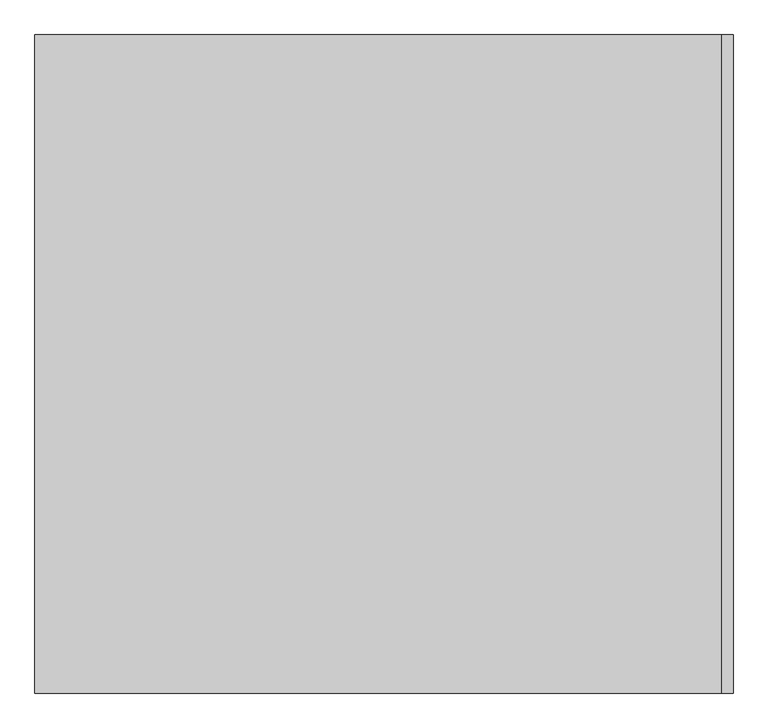
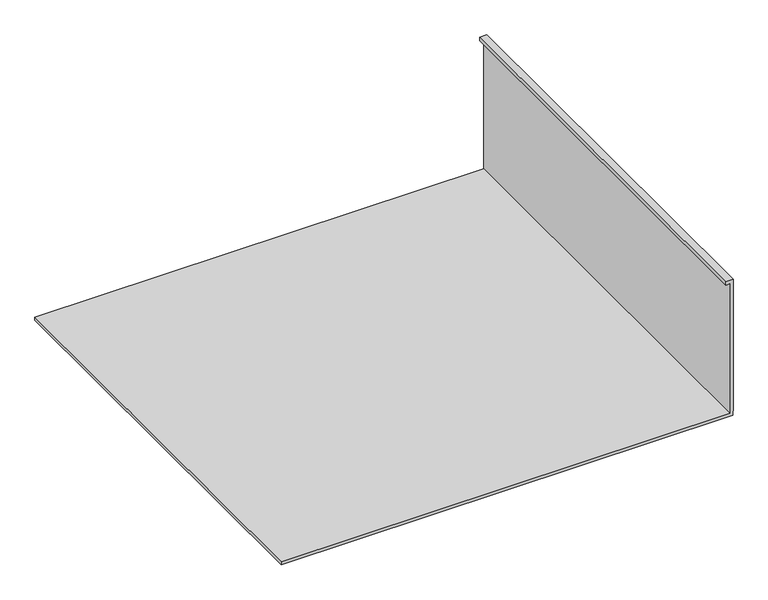
"""IFC4 building model written with IfcOpenShell, lengths in millimetres: proxy geometry, Gypsum022 4491 : Gypsum022 4491."""

from ifc_helpers import new_model, si_unit, frame, origin, place, context, project, spatial, polyline, outline, extrude, source, transform, mapped, element, save


def generic_models_9e6130a8(model_context):
    return source(origin(), model_context, "Body", "SweptSolid", [
        extrude(outline(polyline([(42114.7536708, 4092.7939794), (42098.8786708, 4092.7939794), (42098.8786708, 6190.3030209), (42100.1586708, 6190.3030209), (42100.1586708, 6211.4562048), (42121.3118547, 6211.4562048), (42121.3118547, 6212.7362048), (42771.7862023, 6212.7362048), (42771.7862023, 6178.6035156), (42755.9112023, 6178.6035156), (42755.9112023, 6196.8612048), (42114.7536708, 6196.8612048), (42114.7536708, 4092.7939794)])), frame((0.0, -1052.8908906, 0.0), z_axis=(0.0, 1.0, 0.0), x_axis=(0.0, 0.0, 1.0)), (0.0, 0.0, 1.0), 1999.85),
    ])


if __name__ == "__main__":
    model = new_model("IFC4")
    model_context = context("Model", 3, world=origin())
    ifc_project = project(units=[si_unit("LENGTHUNIT", "METRE", prefix="MILLI")], contexts=[model_context])
    site = spatial("IfcSite", under=ifc_project)
    building = spatial("IfcBuilding", under=site)
    placement = place(None, origin())
    generic_models_shape = generic_models_9e6130a8(model_context)
    element("IfcBuildingElementProxy", 1, Name="Gypsum022 4491 : Gypsum022 4491", ObjectType="Gypsum022 4491 : Gypsum022 4491", at=placement, inside=building, context=model_context, shape_type="MappedRepresentation", body=[
        mapped(generic_models_shape, transform((0.0, 0.0, 0.0), x_axis=(1.0, 0.0, 0.0), y_axis=(0.0, 1.0, 0.0), z_axis=(0.0, 0.0, 1.0))),
    ])
    save(model, "model.ifc")

# Revit data of these elements
# Type "Gypsum022 4491 : Gypsum022 4491"
#   NameOverride = "Gypsum022"
# Element 1 (IfcBuildingElementProxy, "Gypsum022 4491 : Gypsum022 4491")
#   Materials on its faces: "5/8\" GYPSUM BOARD"
# Materials
#   "5/8\" GYPSUM BOARD": class "Unassigned", colour RGB 255 255 255, transparency 0, Cost = 0
